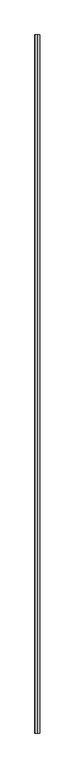
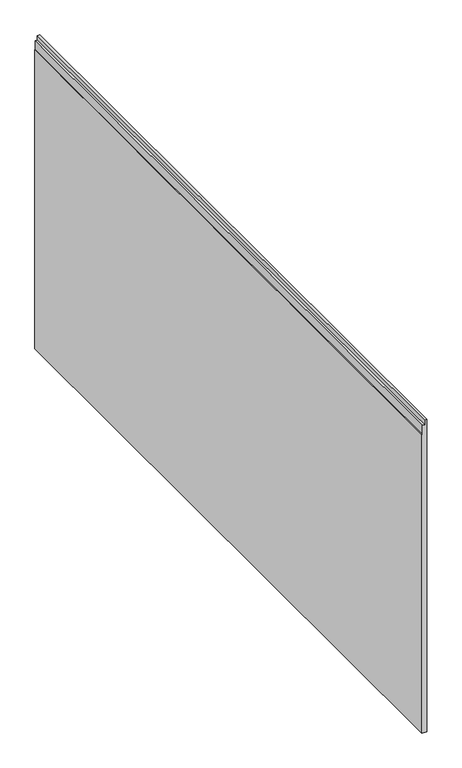
"""IFC4 building model written with IfcOpenShell, lengths in millimetres: proxy geometry, Gypsum025 5573 : Gypsum025 5573."""

from ifc_helpers import new_model, si_unit, frame, origin, place, context, project, spatial, polyline, outline, extrude, source, transform, mapped, element, save


def generic_models_c9eaf26c(model_context):
    return source(origin(), model_context, "Body", "SweptSolid", [
        extrude(outline(polyline([(39807.8954054, 16321.9293635), (39807.8954054, 16336.2168635), (40792.145424, 16336.2168635), (40792.145424, 16329.5993635), (40778.175424, 16329.5993635), (40778.175424, 16323.1993635), (40749.600424, 16323.1993635), (40749.600424, 16321.9293635), (39807.8954054, 16321.9293635)])), frame((0.0, 7982.1484079, 0.0), z_axis=(0.0, 1.0, 0.0), x_axis=(0.0, 0.0, 1.0)), (0.0, 0.0, 1.0), 2000.0),
    ])


if __name__ == "__main__":
    model = new_model("IFC4")
    model_context = context("Model", 3, world=origin())
    ifc_project = project(units=[si_unit("LENGTHUNIT", "METRE", prefix="MILLI")], contexts=[model_context])
    site = spatial("IfcSite", under=ifc_project)
    building = spatial("IfcBuilding", under=site)
    placement = place(None, origin())
    generic_models_shape = generic_models_c9eaf26c(model_context)
    element("IfcBuildingElementProxy", 1, Name="Gypsum025 5573 : Gypsum025 5573", ObjectType="Gypsum025 5573 : Gypsum025 5573", at=placement, inside=building, context=model_context, shape_type="MappedRepresentation", body=[
        mapped(generic_models_shape, transform((0.0, 0.0, 0.0), x_axis=(1.0, 0.0, 0.0), y_axis=(0.0, 1.0, 0.0), z_axis=(0.0, 0.0, 1.0))),
    ])
    save(model, "model.ifc")

# Revit data of these elements
# Type "Gypsum025 5573 : Gypsum025 5573"
#   NameOverride = "Gypsum025"
# Element 1 (IfcBuildingElementProxy, "Gypsum025 5573 : Gypsum025 5573")
#   Materials on its faces: "5/8\" GYPSUM BOARD"
# Materials
#   "5/8\" GYPSUM BOARD": class "Unassigned", colour RGB 214 214 214, transparency 0, Cost = 0
